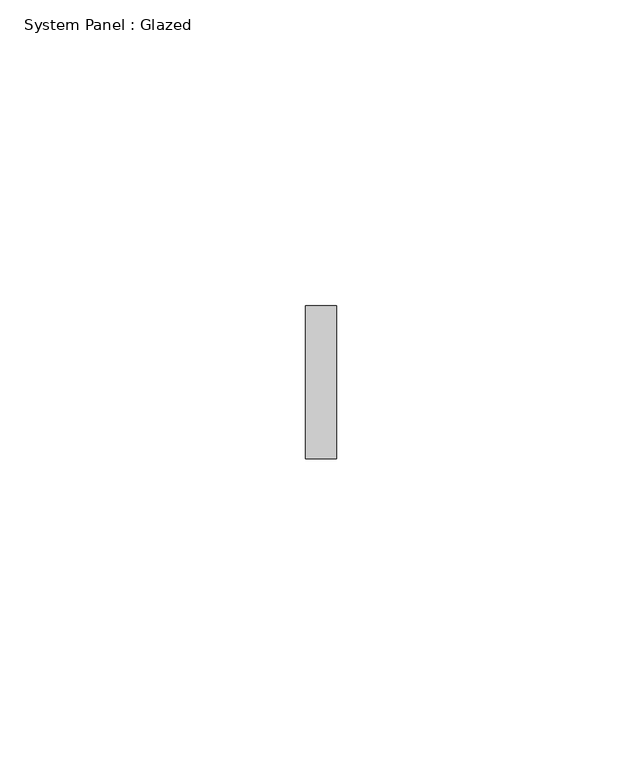
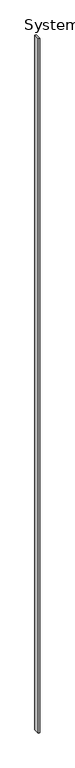
"""IFC4 building model written with IfcOpenShell, lengths in millimetres: plate geometry, System Panel : Glazed."""

from ifc_helpers import new_model, si_unit, origin, origin_with_axes, place, context, project, spatial, polyline, outline, extrude, source, transform, mapped, element, save


def system_panel_glazed_3dc23485(model_context):
    return source(origin(), model_context, "Body", "SweptSolid", [
        extrude(outline(polyline([(2.5, 24.5), (-2.5, 24.5), (-2.5, 49.5), (2.5, 49.5), (2.5, 24.5)])), origin_with_axes(), (0.0, 0.0, 1.0), 3000.0),
    ])


if __name__ == "__main__":
    model = new_model("IFC4")
    model_context = context("Model", 3, world=origin())
    ifc_project = project(units=[si_unit("LENGTHUNIT", "METRE", prefix="MILLI")], contexts=[model_context])
    site = spatial("IfcSite", under=ifc_project)
    building = spatial("IfcBuilding", under=site)
    placement = place(None, origin())
    system_panel_glazed_shape = system_panel_glazed_3dc23485(model_context)
    element("IfcPlate", 1, ObjectType="System Panel : Glazed", at=placement, inside=building, context=model_context, shape_type="MappedRepresentation", body=[
        mapped(system_panel_glazed_shape, transform((0.0, 0.0, 0.0), x_axis=(1.0, 0.0, 0.0), y_axis=(0.0, 1.0, 0.0), z_axis=(0.0, 0.0, 1.0))),
    ])
    save(model, "model.ifc")

# Revit data of these elements
# Element 1 (IfcPlate, "System Panel : Glazed")
#   Materials on its faces: "Glass"
# Materials
#   "Glass": class "Glass", colour RGB 218 227 224, transparency 0.85, Description = "Soda Lime Glass", Cost = 0
